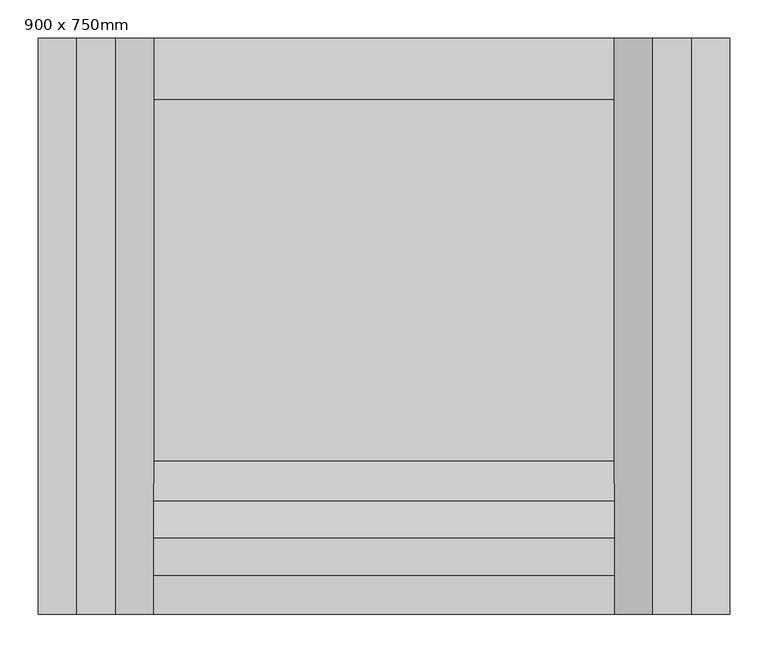
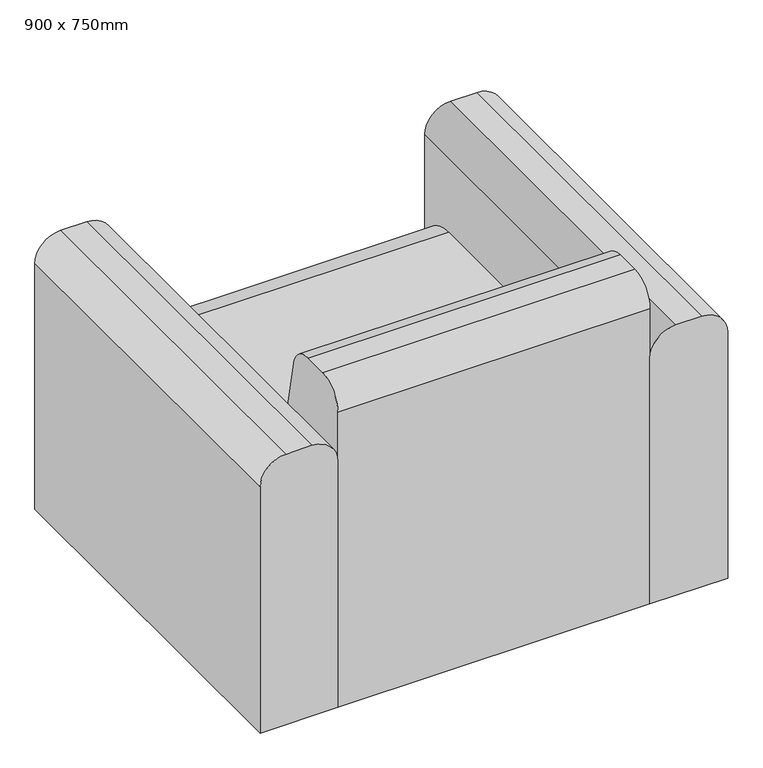
"""IFC4 building model written with IfcOpenShell, lengths in millimetres: furniture geometry, ソファ－I型 : 900 x 750mm."""

import ifcopenshell
import ifcopenshell.guid

model = None  # the IFC model being written
_history = None  # IfcOwnerHistory: only IFC2X3 demands one
_inside = {}  # id of a spatial element -> (the spatial element, [elements in it])
_under = {}  # id of a project, library or spatial element -> (it, [spatial elements below it])
_declared = {}  # id of a project -> (the project, [libraries it declares])
_typed = {}  # id of a type object -> (the type object, [elements of that type])
_made_of = {}  # id of a material, layer set ... -> (it, [elements and type objects made of it])


def new_model(schema):
    """Start an empty IFC model of exactly this schema.

    Asked for "IFC4X3", IfcOpenShell would pick the latest addendum, in which some entities
    have other attributes; the version numbers below select the first issue.
    IFC2X3 requires an IfcOwnerHistory on every rooted entity: one is made here for all.
    """
    global model, _history
    if schema == "IFC4X3":
        model = ifcopenshell.file(schema_version=(4, 3, 0, 0))
    else:
        model = ifcopenshell.file(schema=schema)
    _inside.clear()
    _under.clear()
    _declared.clear()
    _typed.clear()
    _made_of.clear()
    _history = None
    if model.schema == "IFC2X3":
        org = make("IfcOrganization", Name="unknown")
        user = make(
            "IfcPersonAndOrganization",
            ThePerson=make("IfcPerson", FamilyName="unknown"),
            TheOrganization=org,
        )
        app = make(
            "IfcApplication",
            ApplicationDeveloper=org,
            Version="unknown",
            ApplicationFullName="unknown",
            ApplicationIdentifier="unknown",
        )
        _history = make(
            "IfcOwnerHistory",
            OwningUser=user,
            OwningApplication=app,
            ChangeAction="ADDED",
            CreationDate=0,
        )
    return model


def make(cls, **values):
    """One entity of the class cls with the attributes given. An attribute that is None is left unset."""
    return model.create_entity(
        cls, **{name: value for name, value in values.items() if value is not None}
    )


def rooted(cls, **values):
    """An entity with a GlobalId (a new one), such as an element, a storey or a relation."""
    return make(cls, GlobalId=ifcopenshell.guid.new(), OwnerHistory=_history, **values)


def si_unit(unit_type, name, prefix=None):
    """IfcSIUnit, for example si_unit("LENGTHUNIT", "METRE", prefix="MILLI")."""
    return make("IfcSIUnit", UnitType=unit_type, Prefix=prefix, Name=name)


def assignment(units):
    """IfcUnitAssignment: the units of a project."""
    return None if units is None else make("IfcUnitAssignment", Units=units)


def point(xyz):
    """IfcCartesianPoint."""
    return None if xyz is None else make("IfcCartesianPoint", Coordinates=xyz)


def direction(xyz):
    """IfcDirection."""
    return None if xyz is None else make("IfcDirection", DirectionRatios=xyz)


def frame(location, z_axis=None, x_axis=None):
    """IfcAxis2Placement3D, a coordinate frame: its origin and axes. An axis left out is left unset."""
    return make(
        "IfcAxis2Placement3D",
        Location=point(location),
        Axis=direction(z_axis),
        RefDirection=direction(x_axis),
    )


def frame_2d(location, x_axis=None):
    """IfcAxis2Placement2D, a coordinate frame in the plane: its origin and x axis."""
    return make(
        "IfcAxis2Placement2D", Location=point(location), RefDirection=direction(x_axis)
    )


def origin():
    """The frame at (0, 0, 0) with its axes left unset."""
    return frame((0.0, 0.0, 0.0))


def place(relative_to, where):
    """IfcLocalPlacement: puts the frame where relative to a parent placement (None: the world)."""
    return make(
        "IfcLocalPlacement", PlacementRelTo=relative_to, RelativePlacement=where
    )


def context(
    kind, dimensions, precision=None, world=None, true_north=None, identifier=None
):
    """IfcGeometricRepresentationContext, for example the 3D "Model" context."""
    return make(
        "IfcGeometricRepresentationContext",
        ContextIdentifier=identifier,
        ContextType=kind,
        CoordinateSpaceDimension=dimensions,
        Precision=precision,
        WorldCoordinateSystem=world,
        TrueNorth=true_north,
    )


def project(units=None, contexts=None):
    """IfcProject with its units and contexts."""
    return rooted(
        "IfcProject",
        Name="project",
        RepresentationContexts=contexts,
        UnitsInContext=assignment(units),
    )


def spatial(cls, under=None, at=None, **own):
    """A site, building, storey or space (cls), placed at a placement, below another one or the project."""
    s = rooted(cls, ObjectPlacement=at, **own)
    if under is not None:
        _under.setdefault(under.id(), (under, []))[1].append(s)
    return s


def polyline(points):
    """IfcPolyline through the points."""
    return make("IfcPolyline", Points=[point(p) for p in points])


def circle_curve(where, radius):
    """IfcCircle in the frame where."""
    return make("IfcCircle", Position=where, Radius=radius)


def trimmed(basis, trim1, trim2, sense, master):
    """IfcTrimmedCurve: the piece of a basis curve between two trims."""
    return make(
        "IfcTrimmedCurve",
        BasisCurve=basis,
        Trim1=trim1,
        Trim2=trim2,
        SenseAgreement=sense,
        MasterRepresentation=master,
    )


def segment(curve, same_sense, transition):
    """IfcCompositeCurveSegment."""
    return make(
        "IfcCompositeCurveSegment",
        Transition=transition,
        SameSense=same_sense,
        ParentCurve=curve,
    )


def composite_curve(segments, self_intersect=None):
    """IfcCompositeCurve: segments joined end to end."""
    return make("IfcCompositeCurve", Segments=segments, SelfIntersect=self_intersect)


def outline(outer, holes=None, kind="AREA"):
    """IfcArbitraryClosedProfileDef: a profile drawn as a closed curve; with holes, ...WithVoids."""
    if holes is None:
        return make("IfcArbitraryClosedProfileDef", ProfileType=kind, OuterCurve=outer)
    return make(
        "IfcArbitraryProfileDefWithVoids",
        ProfileType=kind,
        OuterCurve=outer,
        InnerCurves=holes,
    )


def extrude(swept, where, along, depth):
    """IfcExtrudedAreaSolid: the profile swept, set in the frame where, extruded along a direction by depth."""
    return make(
        "IfcExtrudedAreaSolid",
        SweptArea=swept,
        Position=where,
        ExtrudedDirection=direction(along),
        Depth=depth,
    )


def shape(context_of_items, identifier, shape_type, items):
    """IfcShapeRepresentation: the items that make up one representation, for example the "Body"."""
    return make(
        "IfcShapeRepresentation",
        ContextOfItems=context_of_items,
        RepresentationIdentifier=identifier,
        RepresentationType=shape_type,
        Items=items,
    )


def source(mapping_origin, context_of_items, identifier, shape_type, items):
    """IfcRepresentationMap: a shape defined once, which mapped items show again and again."""
    return make(
        "IfcRepresentationMap",
        MappingOrigin=mapping_origin,
        MappedRepresentation=shape(context_of_items, identifier, shape_type, items),
    )


def transform(
    local_origin,
    x_axis=None,
    y_axis=None,
    z_axis=None,
    scale=None,
    scale2=None,
    scale3=None,
    uniform=True,
):
    """IfcCartesianTransformationOperator3D, or its non-uniform kind. x_axis, y_axis, z_axis: its Axis1, 2, 3."""
    if uniform:
        return make(
            "IfcCartesianTransformationOperator3D",
            Axis1=direction(x_axis),
            Axis2=direction(y_axis),
            LocalOrigin=point(local_origin),
            Scale=scale,
            Axis3=direction(z_axis),
        )
    return make(
        "IfcCartesianTransformationOperator3DnonUniform",
        Axis1=direction(x_axis),
        Axis2=direction(y_axis),
        LocalOrigin=point(local_origin),
        Scale=scale,
        Axis3=direction(z_axis),
        Scale2=scale2,
        Scale3=scale3,
    )


def mapped(mapping_source, mapping_target):
    """IfcMappedItem: shows the shape of a source again, moved by a transform."""
    return make(
        "IfcMappedItem", MappingSource=mapping_source, MappingTarget=mapping_target
    )


def made_of(thing, what):
    """Note that an element or type object is made of a material, layer set ...; save() writes the relation."""
    if what is not None:
        _made_of.setdefault(what.id(), (what, []))[1].append(thing)
    return thing


def element(
    cls,
    number,
    at=None,
    inside=None,
    cuts=None,
    type_object=None,
    material=None,
    context=None,
    identifier="Body",
    shape_type=None,
    held_by="IfcProductDefinitionShape",
    body=None,
    shapes=None,
    **own,
):
    """One element of the class cls, such as IfcWall. Its Tag is "e" and its number.

    at: its placement. inside: the storey or other place that contains it. cuts: it is an
    opening in that element (IfcRelVoidsElement). A single representation is given by context,
    identifier, shape_type and body (its items); several are given by shapes. held_by: the class
    of the entity that holds the representations. save() writes the other relations.
    """
    e = rooted(cls, Tag="e%d" % number, ObjectPlacement=at, **own)
    if body is not None:
        shapes = [shape(context, identifier, shape_type, body)]
    if shapes is not None:
        e.Representation = make(held_by, Representations=shapes)
    if inside is not None:
        _inside.setdefault(inside.id(), (inside, []))[1].append(e)
    if cuts is not None:
        rooted(
            "IfcRelVoidsElement", RelatingBuildingElement=cuts, RelatedOpeningElement=e
        )
    if type_object is not None:
        _typed.setdefault(type_object.id(), (type_object, []))[1].append(e)
    return made_of(e, material)


def aggregate(whole, parts):
    """IfcRelAggregates: a whole, such as a stair, and the parts it consists of."""
    return rooted("IfcRelAggregates", RelatingObject=whole, RelatedObjects=parts)


def save(model, path):
    """Write the relations noted so far, then the file.

    IfcRelAggregates (storeys below a building ...), IfcRelContainedInSpatialStructure (elements
    in a storey), IfcRelDefinesByType, IfcRelAssociatesMaterial and IfcRelDeclares: one each for
    every whole, place, type object, material and project.
    """
    for whole, parts in _under.values():
        aggregate(whole, parts)
    for where, things in _inside.values():
        rooted(
            "IfcRelContainedInSpatialStructure",
            RelatedElements=things,
            RelatingStructure=where,
        )
    for kind, things in _typed.values():
        rooted("IfcRelDefinesByType", RelatedObjects=things, RelatingType=kind)
    for what, things in _made_of.values():
        rooted("IfcRelAssociatesMaterial", RelatedObjects=things, RelatingMaterial=what)
    for by, libraries in _declared.values():
        rooted("IfcRelDeclares", RelatingContext=by, RelatedDefinitions=libraries)
    model.write(path)


def furniture_900_x_750mm_fd91caf9(model_context):
    return source(origin(), model_context, "Body", "SweptSolid", [
        extrude(outline(composite_curve([segment(trimmed(circle_curve(frame_2d((500.0, -400.0)), 50.0), [point((550.0, -400.0))], [point((500.0, -450.0))], False, "CARTESIAN"), True, "CONTINUOUS"), segment(polyline([(500.0, -450.0), (0.0, -450.0), (0.0, -300.0), (500.0, -300.0)]), True, "CONTINUOUS"), segment(trimmed(circle_curve(frame_2d((500.0, -350.0)), 50.0), [point((500.0, -300.0))], [point((550.0, -350.0))], False, "CARTESIAN"), True, "CONTINUOUS"), segment(polyline([(550.0, -350.0), (550.0, -400.0)]), True, "CONTINUOUS")], self_intersect=False)), frame((0.0, -375.0, 0.0), z_axis=(0.0, 1.0, 0.0), x_axis=(0.0, 0.0, 1.0)), (0.0, 0.0, 1.0), 750.0),
        extrude(outline(composite_curve([segment(polyline([(550.0, 400.0), (550.0, 350.0)]), True, "CONTINUOUS"), segment(trimmed(circle_curve(frame_2d((500.0, 350.0)), 50.0), [point((550.0, 350.0))], [point((500.0, 300.0))], False, "CARTESIAN"), True, "CONTINUOUS"), segment(polyline([(500.0, 300.0), (0.0, 300.0), (0.0, 450.0), (500.0, 450.0)]), True, "CONTINUOUS"), segment(trimmed(circle_curve(frame_2d((500.0, 400.0)), 50.0), [point((500.0, 450.0))], [point((550.0, 400.0))], False, "CARTESIAN"), True, "CONTINUOUS")], self_intersect=False)), frame((0.0, -375.0, 0.0), z_axis=(0.0, 1.0, 0.0), x_axis=(0.0, 0.0, 1.0)), (0.0, 0.0, 1.0), 750.0),
        extrude(outline(composite_curve([segment(polyline([(-226.9611614, 609.8058068), (-175.0, 350.0), (295.0, 350.0)]), True, "CONTINUOUS"), segment(trimmed(circle_curve(frame_2d((295.0, 270.0)), 80.0), [point((295.0, 350.0))], [point((375.0, 270.0))], False, "CARTESIAN"), True, "CONTINUOUS"), segment(polyline([(375.0, 270.0), (375.0, 60.0), (305.0, 60.0), (305.0, 0.0), (-375.0, 0.0), (-375.0, 600.0)]), True, "CONTINUOUS"), segment(trimmed(circle_curve(frame_2d((-325.0, 600.0)), 50.0), [point((-375.0, 600.0))], [point((-325.0, 650.0))], False, "CARTESIAN"), True, "CONTINUOUS"), segment(polyline([(-325.0, 650.0), (-275.9901951, 650.0)]), True, "CONTINUOUS"), segment(trimmed(circle_curve(frame_2d((-275.9901951, 600.0)), 50.0), [point((-275.9901951, 650.0))], [point((-226.9611614, 609.8058068))], False, "CARTESIAN"), True, "CONTINUOUS")], self_intersect=False)), frame((-300.0, 0.0, 0.0), z_axis=(1.0, 0.0, 0.0), x_axis=(0.0, 1.0, 0.0)), (0.0, 0.0, 1.0), 600.0),
    ])


if __name__ == "__main__":
    model = new_model("IFC4")
    model_context = context("Model", 3, world=origin())
    ifc_project = project(units=[si_unit("LENGTHUNIT", "METRE", prefix="MILLI")], contexts=[model_context])
    site = spatial("IfcSite", under=ifc_project)
    building = spatial("IfcBuilding", under=site)
    placement = place(None, origin())
    furniture_900_x_750mm_shape = furniture_900_x_750mm_fd91caf9(model_context)
    element("IfcFurniture", 1, ObjectType="ソファ－I型 : 900 x 750mm", at=placement, inside=building, context=model_context, shape_type="MappedRepresentation", body=[
        mapped(furniture_900_x_750mm_shape, transform((0.0, 0.0, 0.0), x_axis=(1.0, 0.0, 0.0), y_axis=(0.0, 1.0, 0.0), z_axis=(0.0, 0.0, 1.0))),
    ])
    save(model, "model.ifc")

# Revit data of these elements
# Type "ソファ－I型 : 900 x 750mm"
#   Keynote = "12490.Y1"
#   座面高さ = 350 mm
#   幅 = 900 mm
#   奥行き = 750 mm
#   本体 = モチアミ - 無地 - グレー
#   Default Elevation = 0
# Element 1 (IfcFurniture, "ソファ－I型 : 900 x 750mm")
#   Materials on its faces: "モチアミ - 無地 - グレー"
# Materials
#   "モチアミ - 無地 - グレー": class "モチアミ", colour RGB 65 63 65, transparency 0, Cost = 0
